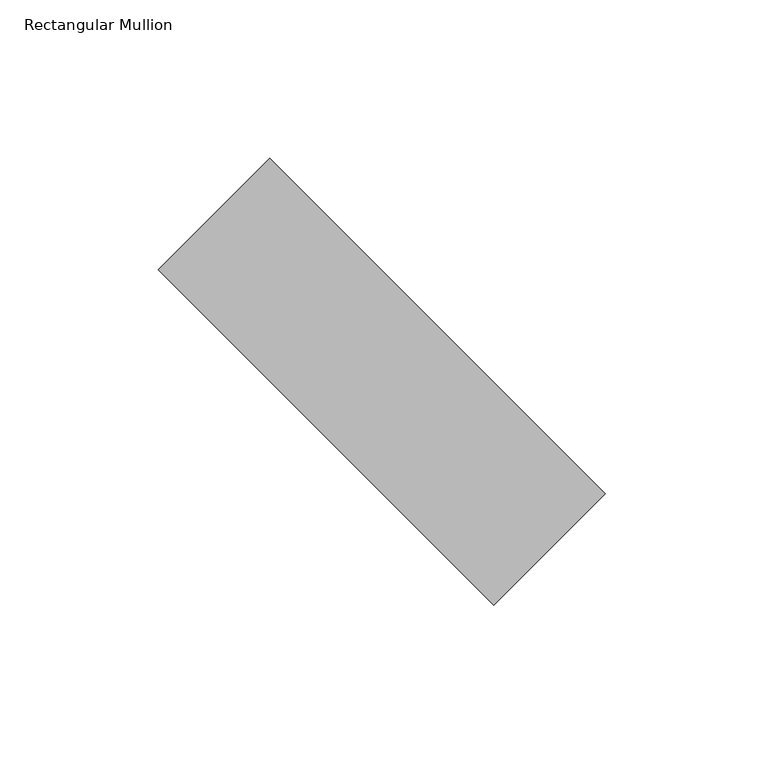
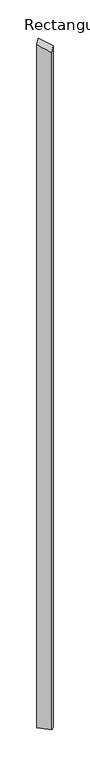
"""IFC4 building model written with IfcOpenShell, lengths in millimetres: member geometry, Rectangular Mullion : tilted mullions."""

from ifc_helpers import new_model, si_unit, origin, place, context, project, spatial, faceted_brep, source, transform, mapped, element, save


def rectangular_mullion_824f0a5b(model_context):
    return source(origin(), model_context, "Body", "Brep", [
        faceted_brep([(-35.3553391, 70.7106781, -7999.8696296), (70.7106781, -35.3553391, -7999.8696296), (35.3553391, -70.7106781, -7999.8696296), (-70.7106781, 35.3553391, -7999.8696296), (-70.7106781, 35.3553391, 9.9721072), (-35.3553391, 70.7106781, 55.0329782), (35.3553391, -70.7106781, -55.0329782), (70.7106781, -35.3553391, -9.9721072)], [[[0, 1, 2, 3]], [[4, 5, 0, 3]], [[6, 4, 3, 2]], [[7, 6, 2, 1]], [[5, 7, 1, 0]], [[5, 4, 6, 7]]]),
    ])


if __name__ == "__main__":
    model = new_model("IFC4")
    model_context = context("Model", 3, world=origin())
    ifc_project = project(units=[si_unit("LENGTHUNIT", "METRE", prefix="MILLI")], contexts=[model_context])
    site = spatial("IfcSite", under=ifc_project)
    building = spatial("IfcBuilding", under=site)
    placement = place(None, origin())
    rectangular_mullion_shape = rectangular_mullion_824f0a5b(model_context)
    element("IfcMember", 1, ObjectType="Rectangular Mullion : tilted mullions", at=placement, inside=building, context=model_context, shape_type="MappedRepresentation", body=[
        mapped(rectangular_mullion_shape, transform((0.0, 0.0, 0.0), x_axis=(1.0, 0.0, 0.0), y_axis=(0.0, 1.0, 0.0), z_axis=(0.0, 0.0, 1.0))),
    ])
    save(model, "model.ifc")

# Revit data of these elements
# Type "Rectangular Mullion : tilted mullions"
#   built-in parameter 1007304 = 0.492126 (stored number, unit not read)
#   built-in parameter 1007301 = 0.082021 (stored number, unit not read)
#   built-in parameter 1007300 = 0.082021 (stored number, unit not read)
# Element 1 (IfcMember, "Rectangular Mullion : tilted mullions")
#   Materials on its faces: "Aluminum"
# Materials
#   "Aluminum": class "Metal", colour RGB 244 244 244, transparency 0, Description = "Aluminum 6061", Cost = 0
